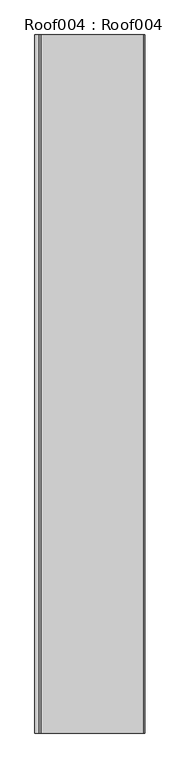
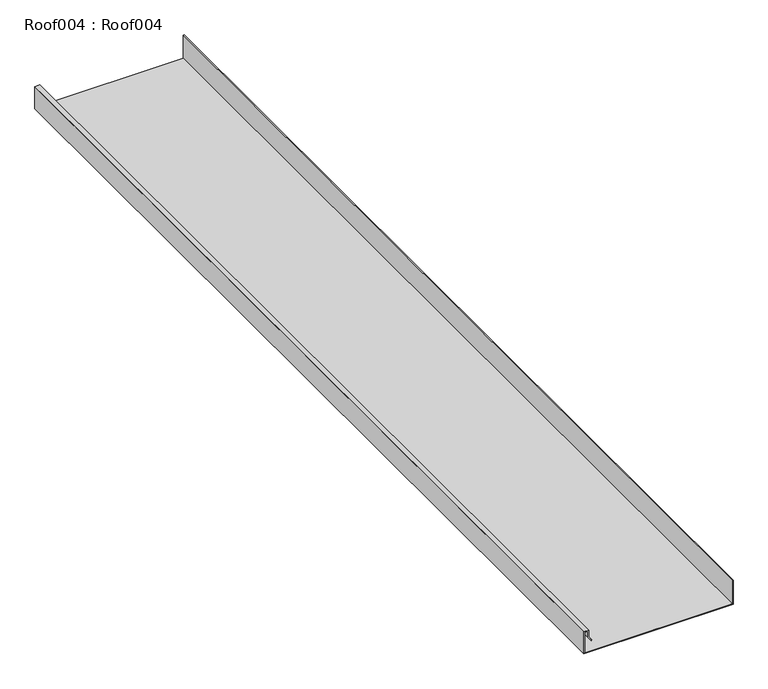
"""IFC4 building model written with IfcOpenShell, lengths in millimetres: proxy geometry, Roof004 : Roof004."""

from ifc_helpers import new_model, si_unit, frame, origin, place, context, project, spatial, polyline, outline, extrude, source, transform, mapped, element, save


def roof004_roof004_a436a50e(model_context):
    return source(origin(), model_context, "Body", "SweptSolid", [
        extrude(outline(polyline([(43494.347072, 17398.7149058), (43484.5384782, 17405.8306285), (43485.7128993, 17407.4494969), (43494.9961263, 17400.7149058), (43509.8322282, 17400.7149058), (43509.8322282, 17390.0401011), (43461.0150407, 17390.0401011), (43461.0150407, 17704.4741831), (43514.7884782, 17704.4741831), (43514.7884782, 17702.4741831), (43463.0150407, 17702.4741831), (43463.0150407, 17392.0401011), (43507.8322282, 17392.0401011), (43507.8322282, 17398.7149058), (43494.347072, 17398.7149058)])), frame((0.0, 7982.1507711, 0.0), z_axis=(0.0, 1.0, 0.0), x_axis=(0.0, 0.0, 1.0)), (0.0, 0.0, 1.0), 2000.0),
    ])


if __name__ == "__main__":
    model = new_model("IFC4")
    model_context = context("Model", 3, world=origin())
    ifc_project = project(units=[si_unit("LENGTHUNIT", "METRE", prefix="MILLI")], contexts=[model_context])
    site = spatial("IfcSite", under=ifc_project)
    building = spatial("IfcBuilding", under=site)
    placement = place(None, origin())
    roof004_roof004_shape = roof004_roof004_a436a50e(model_context)
    element("IfcBuildingElementProxy", 1, Name="Roof004 : Roof004", ObjectType="Roof004 : Roof004", at=placement, inside=building, context=model_context, shape_type="MappedRepresentation", body=[
        mapped(roof004_roof004_shape, transform((0.0, 0.0, 0.0), x_axis=(1.0, 0.0, 0.0), y_axis=(0.0, 1.0, 0.0), z_axis=(0.0, 0.0, 1.0))),
    ])
    save(model, "model.ifc")

# Revit data of these elements
# Type "Roof004 : Roof004"
#   NameOverride = "Roof004"
# Element 1 (IfcBuildingElementProxy, "Roof004 : Roof004")
#   Materials on its faces: "STANDING SEAM METAL ROOF FOLLOW MANU. RECOMMENDED EDGE/TRANSITION DETAILS"
# Materials
#   "STANDING SEAM METAL ROOF FOLLOW MANU. RECOMMENDED EDGE/TRANSITION DETAILS": class "Unassigned", colour RGB 128 128 128, transparency 0, Cost = 0
